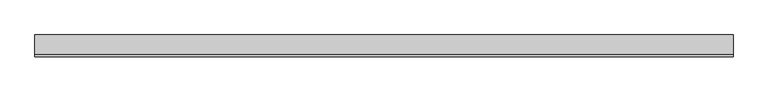
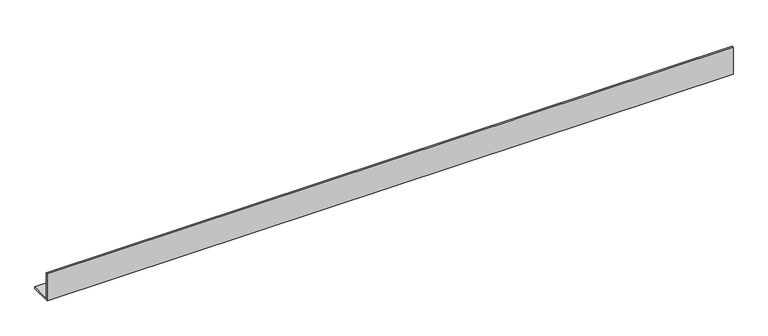
"""IFC4 building model written with IfcOpenShell, lengths in millimetres: proxy geometry, Generic Models 3:Generic Models 1:6:Generic Models 1:6 : Generic Models 3:Generic Models 1:300625:350611:Generic Models 1:6:Generic Models 1:6 : Generic Models 3:Generic Models 1:300625:350611 : Generic Models 3:Generic Models 1:6:Generic Models 1:6 : Generic Models 3:Generic Models 1:300625:350611:4 : Generic Models 3:Generic Models 1:6:Generic Models 1:6 : Generic Models 3:Generic Models 1:300625:350611:Generic Models 1:6:Generic Models 1:6 : Generic Models 3:Generic Models 1:300625:350611 : Generic Models 3:Generic Models 1:6:Generic Models 1:6 : Generic Models 3:Generic Models 1:300625:350611:301824."""

from ifc_helpers import new_model, si_unit, frame, origin, place, context, project, spatial, polyline, outline, extrude, source, transform, mapped, element, save


def generic_models_4ba3d02e(model_context):
    return source(origin(), model_context, "Body", "SweptSolid", [
        extrude(outline(polyline([(-579051.4913841, 0.0), (-579051.4913841, 101.6), (-579045.1413841, 101.6), (-579045.1413841, 6.35), (-578975.2913841, 6.35), (-578975.2913841, 0.0), (-579051.4913841, 0.0)])), frame((599865.8367239, 0.0, 0.0), z_axis=(1.0, 0.0, 0.0), x_axis=(0.0, 1.0, 0.0)), (0.0, 0.0, 1.0), 2438.4),
    ])


if __name__ == "__main__":
    model = new_model("IFC4")
    model_context = context("Model", 3, world=origin())
    ifc_project = project(units=[si_unit("LENGTHUNIT", "METRE", prefix="MILLI")], contexts=[model_context])
    site = spatial("IfcSite", under=ifc_project)
    building = spatial("IfcBuilding", under=site)
    placement = place(None, origin())
    generic_models_shape = generic_models_4ba3d02e(model_context)
    element("IfcBuildingElementProxy", 1, Name="Generic Models 3:Generic Models 1:6:Generic Models 1:6 : Generic Models 3:Generic Models 1:300625:350611:Generic Models 1:6:Generic Models 1:6 : Generic Models 3:Generic Models 1:300625:350611 : Generic Models 3:Generic Models 1:6:Generic Models 1:6 : Generic Models 3:Generic Models 1:300625:350611:4 : Generic Models 3:Generic Models 1:6:Generic Models 1:6 : Generic Models 3:Generic Models 1:300625:350611:Generic Models 1:6:Generic Models 1:6 : Generic Models 3:Generic Models 1:300625:350611 : Generic Models 3:Generic Models 1:6:Generic Models 1:6 : Generic Models 3:Generic Models 1:300625:350611:301824", ObjectType="Generic Models 3:Generic Models 1:6:Generic Models 1:6 : Generic Models 3:Generic Models 1:300625:350611:Generic Models 1:6:Generic Models 1:6 : Generic Models 3:Generic Models 1:300625:350611 : Generic Models 3:Generic Models 1:6:Generic Models 1:6 : Generic Models 3:Generic Models 1:300625:350611:4 : Generic Models 3:Generic Models 1:6:Generic Models 1:6 : Generic Models 3:Generic Models 1:300625:350611:Generic Models 1:6:Generic Models 1:6 : Generic Models 3:Generic Models 1:300625:350611 : Generic Models 3:Generic Models 1:6:Generic Models 1:6 : Generic Models 3:Generic Models 1:300625:350611:301824", at=placement, inside=building, context=model_context, shape_type="MappedRepresentation", body=[
        mapped(generic_models_shape, transform((0.0, 0.0, 0.0), x_axis=(1.0, 0.0, 0.0), y_axis=(0.0, 1.0, 0.0), z_axis=(0.0, 0.0, 1.0))),
    ])
    save(model, "model.ifc")

# Revit data of these elements
# Type "Generic Models 3:Generic Models 1:6:Generic Models 1:6 : Generic Models 3:Generic Models 1:300625:350611:Generic Models 1:6:Generic Models 1:6 : Generic Models 3:Generic Models 1:300625:350611 : Generic Models 3:Generic Models 1:6:Generic Models 1:6 : Generic Models 3:Generic Models 1:300625:350611:4 : Generic Models 3:Generic Models 1:6:Generic Models 1:6 : Generic Models 3:Generic Models 1:300625:350611:Generic Models 1:6:Generic Models 1:6 : Generic Models 3:Generic Models 1:300625:350611 : Generic Models 3:Generic Models 1:6:Generic Models 1:6 : Generic Models 3:Generic Models 1:300625:350611:301824"
#   NameOverride = "Generic Models 3:Generic Models 1:6:Generic Models 1:6 : Generic Models 3:Generic Models 1:300625:350611:Generic Models 1:6:Generic Models 1:6 : Generic Models 3:Generic Models 1:300625:350611 : Generic Models 3:Generic Models 1:6:Generic Models 1:6 : Generic Models 3:Generic Models 1:300625:350611:301824"
#   ObjectTypeOverride = "Generic Models 1:6:Generic Models 1:6 : Generic Models 3:Generic Models 1:300625:350611 : Generic Models 3:Generic Models 1:6:Generic Models 1:6 : Generic Models 3:Generic Models 1:300625:350611"
#   Reference = "Generic Models 1"
#   Tag = "301824"
# Element 1 (IfcBuildingElementProxy, "Generic Models 3:Generic Models 1:6:Generic Models 1:6 : Generic Models 3:Generic Models 1:300625:350611:Generic Models 1:6:Generic Models 1:6 : Generic Models 3:Generic Models 1:300625:350611 : Generic Models 3:Generic Models 1:6:Generic Models 1:6 : Generic Models 3:Generic Models 1:300625:350611:4 : Generic Models 3:Generic Models 1:6:Generic Models 1:6 : Generic Models 3:Generic Models 1:300625:350611:Generic Models 1:6:Generic Models 1:6 : Generic Models 3:Generic Models 1:300625:350611 : Generic Models 3:Generic Models 1:6:Generic Models 1:6 : Generic Models 3:Generic Models 1:300625:350611:301824")
#   Materials on its faces: "6\" Metal Stud Track_1"
# Materials
#   "6\" Metal Stud Track_1": class "Unassigned", colour RGB 120 120 120, transparency 0
